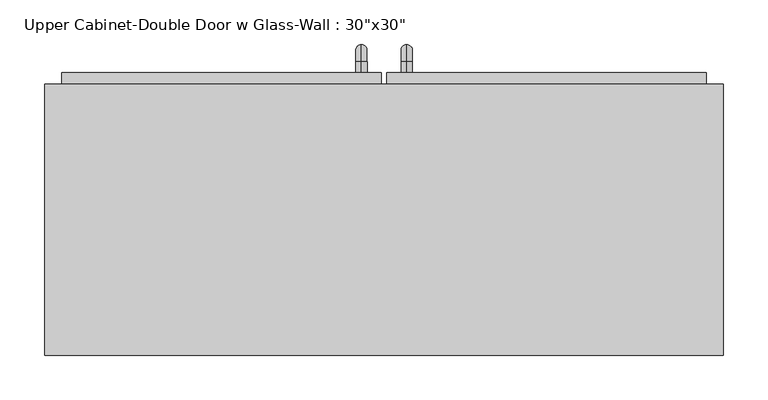
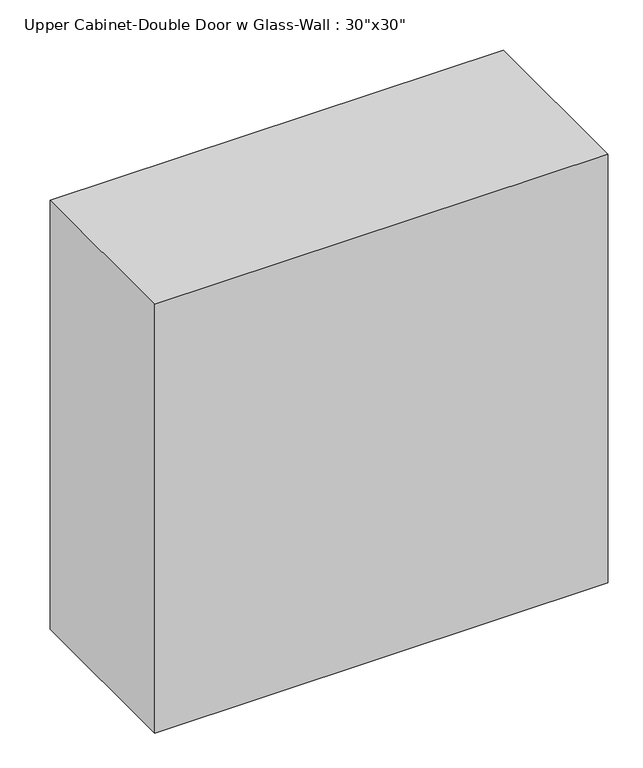
"""IFC4 building model written with IfcOpenShell, lengths in millimetres: furniture geometry."""

from ifc_helpers import new_model, si_unit, point, frame, origin, place, context, project, spatial, polyline, circle_curve, ellipse_curve, trimmed, outline, extrude, faceted_brep, source, transform, mapped, element, save
from ifc_brep_helpers import plane_surface, cylinder_surface, revolved_surface, advanced_brep


def furniture_043e8d7e(model_context):
    return source(origin(), model_context, "Body", "SolidModel", [
        faceted_brep([(-351.2288372, 61.9125, 2590.8), (-351.2288372, 61.9125, 1828.8), (410.7711628, 61.9125, 1828.8), (410.7711628, 61.9125, 2590.8), (-351.2288372, 366.7125, 2590.8), (410.7711628, 366.7125, 2590.8), (410.7711628, 366.7125, 1828.8), (-351.2288372, 366.7125, 1828.8), (-332.1788372, 366.7125, 2571.75), (-332.1788372, 366.7125, 1847.85), (391.7211628, 366.7125, 1847.85), (391.7211628, 366.7125, 2571.75), (391.7211628, 80.9625, 2571.75), (-332.1788372, 80.9625, 2571.75), (391.7211628, 80.9625, 1847.85), (-332.1788372, 80.9625, 1847.85)], [[[0, 1, 2, 3]], [[4, 5, 6, 7], [8, 9, 10, 11]], [[1, 0, 4, 7]], [[2, 1, 7, 6]], [[3, 2, 6, 5]], [[0, 3, 5, 4]], [[8, 11, 12, 13]], [[11, 10, 14, 12]], [[10, 9, 15, 14]], [[9, 8, 13, 15]], [[13, 12, 14, 15]]]),
        advanced_brep(
        [(55.1711628, 379.4125, 1974.85), (55.1711628, 379.4125, 1987.55), (55.1711628, 392.1125, 1974.85), (55.1711628, 392.1125, 1987.55), (55.1711628, 411.1625, 1968.5), (55.1711628, 398.4625, 1968.5), (55.1711628, 398.4625, 1892.3), (55.1711628, 411.1625, 1892.3), (55.1711628, 392.1125, 1873.25), (55.1711628, 392.1125, 1885.95), (55.1711628, 379.4125, 1885.95), (55.1711628, 379.4125, 1873.25)],
        [
            (0, 1, circle_curve(frame((55.1711628, 379.4125, 1981.2), z_axis=(0.0, -1.0, 0.0), x_axis=(0.0, 0.0, -1.0)), 6.35)),
            (1, 0, circle_curve(frame((55.1711628, 379.4125, 1981.2), z_axis=(0.0, -1.0, 0.0), x_axis=(0.0, 0.0, -1.0)), 6.35)),
            (0, 2),
            (2, 3, circle_curve(frame((55.1711628, 392.1125, 1981.2), z_axis=(0.0, -1.0, 0.0), x_axis=(0.0, 0.0, -1.0)), 6.35)),
            (3, 1),
            (3, 2, circle_curve(frame((55.1711628, 392.1125, 1981.2), z_axis=(0.0, -1.0, 0.0), x_axis=(0.0, 0.0, -1.0)), 6.35)),
            (4, 3, circle_curve(frame((55.1711628, 392.1125, 1968.5), z_axis=(1.0, 0.0, 0.0), x_axis=(0.0, 0.0, 1.0)), 19.05)),
            (2, 5, circle_curve(frame((55.1711628, 392.1125, 1968.5), z_axis=(-1.0, 0.0, 0.0), x_axis=(0.0, 0.0, 1.0)), 6.35)),
            (5, 4, circle_curve(frame((55.1711628, 404.8125, 1968.5), z_axis=(0.0, 0.0, 1.0), x_axis=(0.0, -1.0, 0.0)), 6.35)),
            (4, 5, circle_curve(frame((55.1711628, 404.8125, 1968.5), z_axis=(0.0, 0.0, 1.0), x_axis=(0.0, -1.0, 0.0)), 6.35)),
            (5, 6),
            (6, 7, circle_curve(frame((55.1711628, 404.8125, 1892.3), z_axis=(0.0, 0.0, 1.0), x_axis=(0.0, -1.0, 0.0)), 6.35)),
            (7, 4),
            (7, 6, circle_curve(frame((55.1711628, 404.8125, 1892.3), z_axis=(0.0, 0.0, 1.0), x_axis=(0.0, -1.0, 0.0)), 6.35)),
            (8, 7, circle_curve(frame((55.1711628, 392.1125, 1892.3), z_axis=(1.0, 0.0, 0.0), x_axis=(0.0, 1.0, 0.0)), 19.05)),
            (6, 9, circle_curve(frame((55.1711628, 392.1125, 1892.3), z_axis=(-1.0, 0.0, 0.0), x_axis=(0.0, 1.0, 0.0)), 6.35)),
            (9, 8, circle_curve(frame((55.1711628, 392.1125, 1879.6), z_axis=(0.0, 1.0, 0.0), x_axis=(0.0, 0.0, 1.0)), 6.35)),
            (8, 9, circle_curve(frame((55.1711628, 392.1125, 1879.6), z_axis=(0.0, 1.0, 0.0), x_axis=(0.0, 0.0, 1.0)), 6.35)),
            (10, 11, circle_curve(frame((55.1711628, 379.4125, 1879.6), z_axis=(0.0, -1.0, 0.0), x_axis=(0.0, 0.0, 1.0)), 6.35)),
            (11, 10, circle_curve(frame((55.1711628, 379.4125, 1879.6), z_axis=(0.0, -1.0, 0.0), x_axis=(0.0, 0.0, 1.0)), 6.35)),
            (9, 10),
            (11, 8),
        ],
        [
            plane_surface(frame((48.8211628, 379.4125, 1981.2), z_axis=(0.0, -1.0, 0.0), x_axis=(0.0, 0.0, 1.0))),
            cylinder_surface(frame((55.1711628, 379.4125, 1981.2), z_axis=(0.0, -1.0, 0.0), x_axis=(0.0, 0.0, -1.0)), 6.35),
            revolved_surface(trimmed(ellipse_curve(frame((55.1711628, 392.1125, 1981.2), z_axis=(0.0, -1.0, 0.0), x_axis=(0.0, 0.0, -1.0)), 6.35, 6.35), [point((55.1711628, 392.1125, 1974.85))], [point((55.1711628, 392.1125, 1987.55))], True, "CARTESIAN"), (55.1711628, 392.1125, 1968.5), (-1.0, 0.0, 0.0)),
            revolved_surface(trimmed(ellipse_curve(frame((55.1711628, 392.1125, 1981.2), z_axis=(0.0, -1.0, 0.0), x_axis=(0.0, 0.0, -1.0)), 6.35, 6.35), [point((55.1711628, 392.1125, 1987.55))], [point((55.1711628, 392.1125, 1974.85))], True, "CARTESIAN"), (55.1711628, 392.1125, 1968.5), (-1.0, 0.0, 0.0)),
            cylinder_surface(frame((55.1711628, 404.8125, 1968.5), z_axis=(0.0, 0.0, 1.0), x_axis=(0.0, -1.0, 0.0)), 6.35),
            revolved_surface(trimmed(ellipse_curve(frame((55.1711628, 404.8125, 1892.3), z_axis=(0.0, 0.0, 1.0), x_axis=(0.0, -1.0, 0.0)), 6.35, 6.35), [point((55.1711628, 398.4625, 1892.3))], [point((55.1711628, 411.1625, 1892.3))], True, "CARTESIAN"), (55.1711628, 392.1125, 1892.3), (-1.0, 0.0, 0.0)),
            revolved_surface(trimmed(ellipse_curve(frame((55.1711628, 404.8125, 1892.3), z_axis=(0.0, 0.0, 1.0), x_axis=(0.0, -1.0, 0.0)), 6.35, 6.35), [point((55.1711628, 411.1625, 1892.3))], [point((55.1711628, 398.4625, 1892.3))], True, "CARTESIAN"), (55.1711628, 392.1125, 1892.3), (-1.0, 0.0, 0.0)),
            plane_surface(frame((48.8211628, 379.4125, 1879.6), z_axis=(0.0, -1.0, 0.0), x_axis=(0.0, 0.0, -1.0))),
            cylinder_surface(frame((55.1711628, 392.1125, 1879.6), z_axis=(0.0, 1.0, 0.0), x_axis=(0.0, 0.0, 1.0)), 6.35),
        ],
        [
            (0, [[1, 2]]),
            (1, [[-1, 3, 4, 5]]),
            (1, [[-2, -5, 6, -3]]),
            (2, [[7, -4, 8, 9]]),
            (3, [[-8, -6, -7, 10]]),
            (4, [[-9, 11, 12, 13]]),
            (4, [[-10, -13, 14, -11]]),
            (5, [[15, -12, 16, 17]]),
            (6, [[-16, -14, -15, 18]]),
            (7, [[19, 20]]),
            (8, [[-17, 21, -20, 22]]),
            (8, [[-18, -22, -19, -21]]),
        ],
    ),
        advanced_brep(
        [(4.3711628, 379.4125, 1974.85), (4.3711628, 379.4125, 1987.55), (4.3711628, 392.1125, 1974.85), (4.3711628, 392.1125, 1987.55), (4.3711628, 411.1625, 1968.5), (4.3711628, 398.4625, 1968.5), (4.3711628, 398.4625, 1892.3), (4.3711628, 411.1625, 1892.3), (4.3711628, 392.1125, 1873.25), (4.3711628, 392.1125, 1885.95), (4.3711628, 379.4125, 1885.95), (4.3711628, 379.4125, 1873.25)],
        [
            (0, 1, circle_curve(frame((4.3711628, 379.4125, 1981.2), z_axis=(0.0, -1.0, 0.0), x_axis=(0.0, 0.0, 1.0)), 6.35)),
            (1, 0, circle_curve(frame((4.3711628, 379.4125, 1981.2), z_axis=(0.0, -1.0, 0.0), x_axis=(0.0, 0.0, 1.0)), 6.35)),
            (0, 2),
            (2, 3, circle_curve(frame((4.3711628, 392.1125, 1981.2), z_axis=(0.0, -1.0, 0.0), x_axis=(0.0, 0.0, 1.0)), 6.35)),
            (3, 1),
            (3, 2, circle_curve(frame((4.3711628, 392.1125, 1981.2), z_axis=(0.0, -1.0, 0.0), x_axis=(0.0, 0.0, 1.0)), 6.35)),
            (4, 3, circle_curve(frame((4.3711628, 392.1125, 1968.5), z_axis=(1.0, 0.0, 0.0), x_axis=(0.0, 0.0, 1.0)), 19.05)),
            (2, 5, circle_curve(frame((4.3711628, 392.1125, 1968.5), z_axis=(-1.0, 0.0, 0.0), x_axis=(0.0, 0.0, 1.0)), 6.35)),
            (5, 4, circle_curve(frame((4.3711628, 404.8125, 1968.5), z_axis=(0.0, 0.0, 1.0), x_axis=(0.0, 1.0, 0.0)), 6.35)),
            (4, 5, circle_curve(frame((4.3711628, 404.8125, 1968.5), z_axis=(0.0, 0.0, 1.0), x_axis=(0.0, 1.0, 0.0)), 6.35)),
            (5, 6),
            (6, 7, circle_curve(frame((4.3711628, 404.8125, 1892.3), z_axis=(0.0, 0.0, 1.0), x_axis=(0.0, 1.0, 0.0)), 6.35)),
            (7, 4),
            (7, 6, circle_curve(frame((4.3711628, 404.8125, 1892.3), z_axis=(0.0, 0.0, 1.0), x_axis=(0.0, 1.0, 0.0)), 6.35)),
            (8, 7, circle_curve(frame((4.3711628, 392.1125, 1892.3), z_axis=(1.0, 0.0, 0.0), x_axis=(0.0, 1.0, 0.0)), 19.05)),
            (6, 9, circle_curve(frame((4.3711628, 392.1125, 1892.3), z_axis=(-1.0, 0.0, 0.0), x_axis=(0.0, 1.0, 0.0)), 6.35)),
            (9, 8, circle_curve(frame((4.3711628, 392.1125, 1879.6), z_axis=(0.0, 1.0, 0.0), x_axis=(0.0, 0.0, -1.0)), 6.35)),
            (8, 9, circle_curve(frame((4.3711628, 392.1125, 1879.6), z_axis=(0.0, 1.0, 0.0), x_axis=(0.0, 0.0, -1.0)), 6.35)),
            (10, 11, circle_curve(frame((4.3711628, 379.4125, 1879.6), z_axis=(0.0, -1.0, 0.0), x_axis=(0.0, 0.0, -1.0)), 6.35)),
            (11, 10, circle_curve(frame((4.3711628, 379.4125, 1879.6), z_axis=(0.0, -1.0, 0.0), x_axis=(0.0, 0.0, -1.0)), 6.35)),
            (9, 10),
            (11, 8),
        ],
        [
            plane_surface(frame((-1.9788372, 379.4125, 1981.2), z_axis=(0.0, -1.0, 0.0), x_axis=(0.0, 0.0, 1.0))),
            cylinder_surface(frame((4.3711628, 379.4125, 1981.2), z_axis=(0.0, -1.0, 0.0), x_axis=(0.0, 0.0, 1.0)), 6.35),
            revolved_surface(trimmed(ellipse_curve(frame((4.3711628, 392.1125, 1981.2), z_axis=(0.0, -1.0, 0.0), x_axis=(0.0, 0.0, 1.0)), 6.35, 6.35), [point((4.3711628, 392.1125, 1974.85))], [point((4.3711628, 392.1125, 1987.55))], True, "CARTESIAN"), (4.3711628, 392.1125, 1968.5), (-1.0, 0.0, 0.0)),
            revolved_surface(trimmed(ellipse_curve(frame((4.3711628, 392.1125, 1981.2), z_axis=(0.0, -1.0, 0.0), x_axis=(0.0, 0.0, 1.0)), 6.35, 6.35), [point((4.3711628, 392.1125, 1987.55))], [point((4.3711628, 392.1125, 1974.85))], True, "CARTESIAN"), (4.3711628, 392.1125, 1968.5), (-1.0, 0.0, 0.0)),
            cylinder_surface(frame((4.3711628, 404.8125, 1968.5), z_axis=(0.0, 0.0, 1.0), x_axis=(0.0, 1.0, 0.0)), 6.35),
            revolved_surface(trimmed(ellipse_curve(frame((4.3711628, 404.8125, 1892.3), z_axis=(0.0, 0.0, 1.0), x_axis=(0.0, 1.0, 0.0)), 6.35, 6.35), [point((4.3711628, 398.4625, 1892.3))], [point((4.3711628, 411.1625, 1892.3))], True, "CARTESIAN"), (4.3711628, 392.1125, 1892.3), (-1.0, 0.0, 0.0)),
            revolved_surface(trimmed(ellipse_curve(frame((4.3711628, 404.8125, 1892.3), z_axis=(0.0, 0.0, 1.0), x_axis=(0.0, 1.0, 0.0)), 6.35, 6.35), [point((4.3711628, 411.1625, 1892.3))], [point((4.3711628, 398.4625, 1892.3))], True, "CARTESIAN"), (4.3711628, 392.1125, 1892.3), (-1.0, 0.0, 0.0)),
            plane_surface(frame((-1.9788372, 379.4125, 1879.6), z_axis=(0.0, -1.0, 0.0), x_axis=(0.0, 0.0, -1.0))),
            cylinder_surface(frame((4.3711628, 392.1125, 1879.6), z_axis=(0.0, 1.0, 0.0), x_axis=(0.0, 0.0, -1.0)), 6.35),
        ],
        [
            (0, [[1, 2]]),
            (1, [[-1, 3, 4, 5]]),
            (1, [[-2, -5, 6, -3]]),
            (2, [[7, -4, 8, 9]]),
            (3, [[-8, -6, -7, 10]]),
            (4, [[-9, 11, 12, 13]]),
            (4, [[-10, -13, 14, -11]]),
            (5, [[15, -12, 16, 17]]),
            (6, [[-16, -14, -15, 18]]),
            (7, [[19, 20]]),
            (8, [[-17, 21, -20, 22]]),
            (8, [[-18, -22, -19, -21]]),
        ],
    ),
        extrude(outline(polyline([(64.6961628, 360.3625), (359.9711628, 360.3625), (359.9711628, 354.0125), (64.6961628, 354.0125), (64.6961628, 360.3625)])), frame((0.0, 0.0, 1879.6), z_axis=(0.0, 0.0, 1.0), x_axis=(1.0, 0.0, 0.0)), (0.0, 0.0, 1.0), 660.4),
        extrude(outline(polyline([(-300.4288372, 360.3625), (-5.1538372, 360.3625), (-5.1538372, 354.0125), (-300.4288372, 354.0125), (-300.4288372, 360.3625)])), frame((0.0, 0.0, 1879.6), z_axis=(0.0, 0.0, 1.0), x_axis=(1.0, 0.0, 0.0)), (0.0, 0.0, 1.0), 660.4),
        extrude(outline(polyline([(2571.75, 32.9461628), (1847.85, 32.9461628), (1847.85, 391.7211628), (2571.75, 391.7211628), (2571.75, 32.9461628)]), holes=[polyline([(1879.6, 64.6961628), (2540.0, 64.6961628), (2540.0, 359.9711628), (1879.6, 359.9711628), (1879.6, 64.6961628)])]), frame((0.0, 347.6625, 0.0), z_axis=(0.0, 1.0, 0.0), x_axis=(0.0, 0.0, 1.0)), (0.0, 0.0, 1.0), 31.75),
        extrude(outline(polyline([(1847.85, -332.1788372), (1847.85, 26.5961628), (2571.75, 26.5961628), (2571.75, -332.1788372), (1847.85, -332.1788372)]), holes=[polyline([(2540.0, -5.1538372), (1879.6, -5.1538372), (1879.6, -300.4288372), (2540.0, -300.4288372), (2540.0, -5.1538372)])]), frame((0.0, 347.6625, 0.0), z_axis=(0.0, 1.0, 0.0), x_axis=(0.0, 0.0, 1.0)), (0.0, 0.0, 1.0), 31.75),
    ])


if __name__ == "__main__":
    model = new_model("IFC4")
    model_context = context("Model", 3, world=origin())
    ifc_project = project(units=[si_unit("LENGTHUNIT", "METRE", prefix="MILLI")], contexts=[model_context])
    site = spatial("IfcSite", under=ifc_project)
    building = spatial("IfcBuilding", under=site)
    placement = place(None, origin())
    furniture_shape = furniture_043e8d7e(model_context)
    element("IfcFurniture", 1, ObjectType="Upper Cabinet-Double Door w Glass-Wall : 30\"x30\"", at=placement, inside=building, context=model_context, shape_type="MappedRepresentation", body=[
        mapped(furniture_shape, transform((0.0, 0.0, 0.0), x_axis=(1.0, 0.0, 0.0), y_axis=(0.0, 1.0, 0.0), z_axis=(0.0, 0.0, 1.0))),
    ])
    save(model, "model.ifc")

# Revit data of these elements
# Type "Upper Cabinet-Double Door w Glass-Wall : 30\"x30\""
#   Assembly Code = "C1030410"
#   Depth = 1' - 0"
#   Height = 2' - 6"
#   Top Of Cabinet = 8' - 6"
#   Width = 2' - 6"
#   COBie.Type = no
#   Cabinet Material = none
#   Door/Drawer Material = none
#   Handle Material = Cabinets - Handles
#   Panel Material = Glass
# Element 1 (IfcFurniture, "Upper Cabinet-Double Door w Glass-Wall : 30\"x30\"")
#   Materials on its faces: "Cabinets", "Cabinets - Handles", "Glass"
# Materials
#   "Cabinets - Handles": class "Metal", colour RGB 57 57 57, transparency 0
#   "Glass": class "Glass", colour RGB 0 128 192, transparency 0.75, Description = "Soda Lime Glass", Cost = 0
#   "Cabinets": class "Miscellaneous", colour RGB 249 249 249, transparency 0
